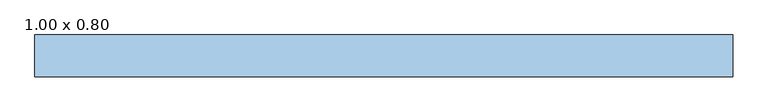
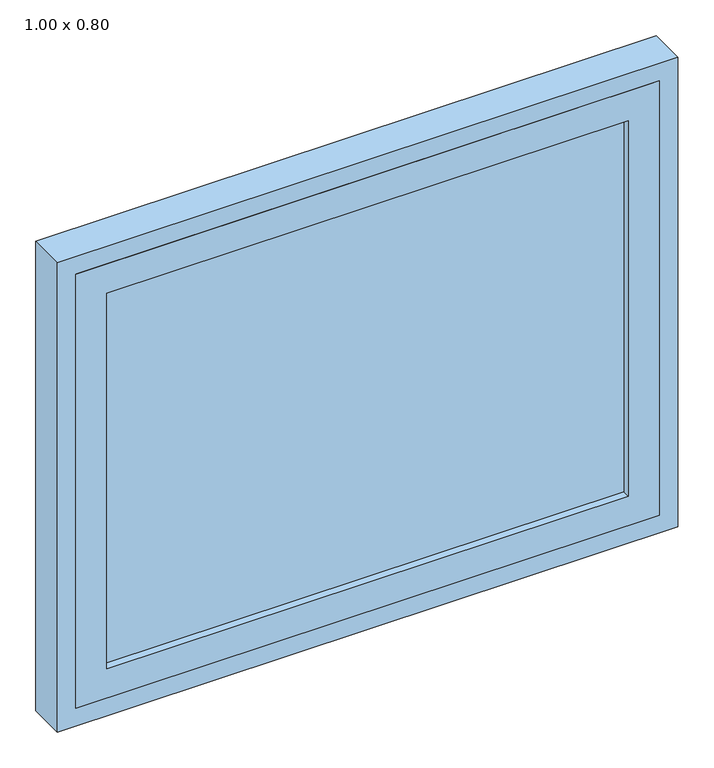
"""IFC4 building model written with IfcOpenShell, lengths in millimetres: window geometry, CC_JANELA MAXIM-AR_1 FOLHA VIDRO : 1.00 x 0.80."""

import ifcopenshell
import ifcopenshell.guid

model = None  # the IFC model being written
_history = None  # IfcOwnerHistory: only IFC2X3 demands one
_inside = {}  # id of a spatial element -> (the spatial element, [elements in it])
_under = {}  # id of a project, library or spatial element -> (it, [spatial elements below it])
_declared = {}  # id of a project -> (the project, [libraries it declares])
_typed = {}  # id of a type object -> (the type object, [elements of that type])
_made_of = {}  # id of a material, layer set ... -> (it, [elements and type objects made of it])


def new_model(schema):
    """Start an empty IFC model of exactly this schema.

    Asked for "IFC4X3", IfcOpenShell would pick the latest addendum, in which some entities
    have other attributes; the version numbers below select the first issue.
    IFC2X3 requires an IfcOwnerHistory on every rooted entity: one is made here for all.
    """
    global model, _history
    if schema == "IFC4X3":
        model = ifcopenshell.file(schema_version=(4, 3, 0, 0))
    else:
        model = ifcopenshell.file(schema=schema)
    _inside.clear()
    _under.clear()
    _declared.clear()
    _typed.clear()
    _made_of.clear()
    _history = None
    if model.schema == "IFC2X3":
        org = make("IfcOrganization", Name="unknown")
        user = make(
            "IfcPersonAndOrganization",
            ThePerson=make("IfcPerson", FamilyName="unknown"),
            TheOrganization=org,
        )
        app = make(
            "IfcApplication",
            ApplicationDeveloper=org,
            Version="unknown",
            ApplicationFullName="unknown",
            ApplicationIdentifier="unknown",
        )
        _history = make(
            "IfcOwnerHistory",
            OwningUser=user,
            OwningApplication=app,
            ChangeAction="ADDED",
            CreationDate=0,
        )
    return model


def make(cls, **values):
    """One entity of the class cls with the attributes given. An attribute that is None is left unset."""
    return model.create_entity(
        cls, **{name: value for name, value in values.items() if value is not None}
    )


def rooted(cls, **values):
    """An entity with a GlobalId (a new one), such as an element, a storey or a relation."""
    return make(cls, GlobalId=ifcopenshell.guid.new(), OwnerHistory=_history, **values)


def si_unit(unit_type, name, prefix=None):
    """IfcSIUnit, for example si_unit("LENGTHUNIT", "METRE", prefix="MILLI")."""
    return make("IfcSIUnit", UnitType=unit_type, Prefix=prefix, Name=name)


def assignment(units):
    """IfcUnitAssignment: the units of a project."""
    return None if units is None else make("IfcUnitAssignment", Units=units)


def point(xyz):
    """IfcCartesianPoint."""
    return None if xyz is None else make("IfcCartesianPoint", Coordinates=xyz)


def direction(xyz):
    """IfcDirection."""
    return None if xyz is None else make("IfcDirection", DirectionRatios=xyz)


def frame(location, z_axis=None, x_axis=None):
    """IfcAxis2Placement3D, a coordinate frame: its origin and axes. An axis left out is left unset."""
    return make(
        "IfcAxis2Placement3D",
        Location=point(location),
        Axis=direction(z_axis),
        RefDirection=direction(x_axis),
    )


def origin():
    """The frame at (0, 0, 0) with its axes left unset."""
    return frame((0.0, 0.0, 0.0))


def place(relative_to, where):
    """IfcLocalPlacement: puts the frame where relative to a parent placement (None: the world)."""
    return make(
        "IfcLocalPlacement", PlacementRelTo=relative_to, RelativePlacement=where
    )


def context(
    kind, dimensions, precision=None, world=None, true_north=None, identifier=None
):
    """IfcGeometricRepresentationContext, for example the 3D "Model" context."""
    return make(
        "IfcGeometricRepresentationContext",
        ContextIdentifier=identifier,
        ContextType=kind,
        CoordinateSpaceDimension=dimensions,
        Precision=precision,
        WorldCoordinateSystem=world,
        TrueNorth=true_north,
    )


def project(units=None, contexts=None):
    """IfcProject with its units and contexts."""
    return rooted(
        "IfcProject",
        Name="project",
        RepresentationContexts=contexts,
        UnitsInContext=assignment(units),
    )


def spatial(cls, under=None, at=None, **own):
    """A site, building, storey or space (cls), placed at a placement, below another one or the project."""
    s = rooted(cls, ObjectPlacement=at, **own)
    if under is not None:
        _under.setdefault(under.id(), (under, []))[1].append(s)
    return s


def polyline(points):
    """IfcPolyline through the points."""
    return make("IfcPolyline", Points=[point(p) for p in points])


def outline(outer, holes=None, kind="AREA"):
    """IfcArbitraryClosedProfileDef: a profile drawn as a closed curve; with holes, ...WithVoids."""
    if holes is None:
        return make("IfcArbitraryClosedProfileDef", ProfileType=kind, OuterCurve=outer)
    return make(
        "IfcArbitraryProfileDefWithVoids",
        ProfileType=kind,
        OuterCurve=outer,
        InnerCurves=holes,
    )


def extrude(swept, where, along, depth):
    """IfcExtrudedAreaSolid: the profile swept, set in the frame where, extruded along a direction by depth."""
    return make(
        "IfcExtrudedAreaSolid",
        SweptArea=swept,
        Position=where,
        ExtrudedDirection=direction(along),
        Depth=depth,
    )


def shape(context_of_items, identifier, shape_type, items):
    """IfcShapeRepresentation: the items that make up one representation, for example the "Body"."""
    return make(
        "IfcShapeRepresentation",
        ContextOfItems=context_of_items,
        RepresentationIdentifier=identifier,
        RepresentationType=shape_type,
        Items=items,
    )


def source(mapping_origin, context_of_items, identifier, shape_type, items):
    """IfcRepresentationMap: a shape defined once, which mapped items show again and again."""
    return make(
        "IfcRepresentationMap",
        MappingOrigin=mapping_origin,
        MappedRepresentation=shape(context_of_items, identifier, shape_type, items),
    )


def transform(
    local_origin,
    x_axis=None,
    y_axis=None,
    z_axis=None,
    scale=None,
    scale2=None,
    scale3=None,
    uniform=True,
):
    """IfcCartesianTransformationOperator3D, or its non-uniform kind. x_axis, y_axis, z_axis: its Axis1, 2, 3."""
    if uniform:
        return make(
            "IfcCartesianTransformationOperator3D",
            Axis1=direction(x_axis),
            Axis2=direction(y_axis),
            LocalOrigin=point(local_origin),
            Scale=scale,
            Axis3=direction(z_axis),
        )
    return make(
        "IfcCartesianTransformationOperator3DnonUniform",
        Axis1=direction(x_axis),
        Axis2=direction(y_axis),
        LocalOrigin=point(local_origin),
        Scale=scale,
        Axis3=direction(z_axis),
        Scale2=scale2,
        Scale3=scale3,
    )


def mapped(mapping_source, mapping_target):
    """IfcMappedItem: shows the shape of a source again, moved by a transform."""
    return make(
        "IfcMappedItem", MappingSource=mapping_source, MappingTarget=mapping_target
    )


def made_of(thing, what):
    """Note that an element or type object is made of a material, layer set ...; save() writes the relation."""
    if what is not None:
        _made_of.setdefault(what.id(), (what, []))[1].append(thing)
    return thing


def element(
    cls,
    number,
    at=None,
    inside=None,
    cuts=None,
    type_object=None,
    material=None,
    context=None,
    identifier="Body",
    shape_type=None,
    held_by="IfcProductDefinitionShape",
    body=None,
    shapes=None,
    **own,
):
    """One element of the class cls, such as IfcWall. Its Tag is "e" and its number.

    at: its placement. inside: the storey or other place that contains it. cuts: it is an
    opening in that element (IfcRelVoidsElement). A single representation is given by context,
    identifier, shape_type and body (its items); several are given by shapes. held_by: the class
    of the entity that holds the representations. save() writes the other relations.
    """
    e = rooted(cls, Tag="e%d" % number, ObjectPlacement=at, **own)
    if body is not None:
        shapes = [shape(context, identifier, shape_type, body)]
    if shapes is not None:
        e.Representation = make(held_by, Representations=shapes)
    if inside is not None:
        _inside.setdefault(inside.id(), (inside, []))[1].append(e)
    if cuts is not None:
        rooted(
            "IfcRelVoidsElement", RelatingBuildingElement=cuts, RelatedOpeningElement=e
        )
    if type_object is not None:
        _typed.setdefault(type_object.id(), (type_object, []))[1].append(e)
    return made_of(e, material)


def aggregate(whole, parts):
    """IfcRelAggregates: a whole, such as a stair, and the parts it consists of."""
    return rooted("IfcRelAggregates", RelatingObject=whole, RelatedObjects=parts)


def save(model, path):
    """Write the relations noted so far, then the file.

    IfcRelAggregates (storeys below a building ...), IfcRelContainedInSpatialStructure (elements
    in a storey), IfcRelDefinesByType, IfcRelAssociatesMaterial and IfcRelDeclares: one each for
    every whole, place, type object, material and project.
    """
    for whole, parts in _under.values():
        aggregate(whole, parts)
    for where, things in _inside.values():
        rooted(
            "IfcRelContainedInSpatialStructure",
            RelatedElements=things,
            RelatingStructure=where,
        )
    for kind, things in _typed.values():
        rooted("IfcRelDefinesByType", RelatedObjects=things, RelatingType=kind)
    for what, things in _made_of.values():
        rooted("IfcRelAssociatesMaterial", RelatedObjects=things, RelatingMaterial=what)
    for by, libraries in _declared.values():
        rooted("IfcRelDeclares", RelatingContext=by, RelatedDefinitions=libraries)
    model.write(path)


def window_1_00_x_0_80_3e14d2bc(model_context):
    return source(origin(), model_context, "Body", "SweptSolid", [
        extrude(outline(polyline([(-420.0, -87.5), (-420.0, -82.5), (420.0, -82.5), (420.0, -87.5), (-420.0, -87.5)])), frame((0.0, 0.0, 1780.0), z_axis=(0.0, 0.0, 1.0), x_axis=(1.0, 0.0, 0.0)), (0.0, 0.0, 1.0), 640.0),
        extrude(outline(polyline([(2470.0, -470.0), (1730.0, -470.0), (1730.0, 470.0), (2470.0, 470.0), (2470.0, -470.0)]), holes=[polyline([(2420.0, 420.0), (1780.0, 420.0), (1780.0, -420.0), (2420.0, -420.0), (2420.0, 420.0)])]), frame((0.0, -100.0, 0.0), z_axis=(0.0, 1.0, 0.0), x_axis=(0.0, 0.0, 1.0)), (0.0, 0.0, 1.0), 30.0),
        extrude(outline(polyline([(1700.0, 500.0), (2500.0, 500.0), (2500.0, -500.0), (1700.0, -500.0), (1700.0, 500.0)]), holes=[polyline([(1730.0, -470.0), (2470.0, -470.0), (2470.0, 470.0), (1730.0, 470.0), (1730.0, -470.0)])]), frame((0.0, -100.0, 0.0), z_axis=(0.0, 1.0, 0.0), x_axis=(0.0, 0.0, 1.0)), (0.0, 0.0, 1.0), 60.0),
    ])


if __name__ == "__main__":
    model = new_model("IFC4")
    model_context = context("Model", 3, world=origin())
    ifc_project = project(units=[si_unit("LENGTHUNIT", "METRE", prefix="MILLI")], contexts=[model_context])
    site = spatial("IfcSite", under=ifc_project)
    building = spatial("IfcBuilding", under=site)
    placement = place(None, origin())
    window_1_00_x_0_80_shape = window_1_00_x_0_80_3e14d2bc(model_context)
    element("IfcWindow", 1, ObjectType="CC_JANELA MAXIM-AR_1 FOLHA VIDRO : 1.00 x 0.80", at=placement, inside=building, context=model_context, shape_type="MappedRepresentation", body=[
        mapped(window_1_00_x_0_80_shape, transform((0.0, 0.0, 0.0), x_axis=(1.0, 0.0, 0.0), y_axis=(0.0, 1.0, 0.0), z_axis=(0.0, 0.0, 1.0))),
    ])
    save(model, "model.ifc")

# Revit data of these elements
# Type "CC_JANELA MAXIM-AR_1 FOLHA VIDRO : 1.00 x 0.80"
#   Type Mark = "J7"
#   Site = "www.construir.arq.br"
#   Empresa = "Cursos Construir"
#   Description = "JANELA MAXIM-AR 1 FOLHA VIDRO"
#   Criado Por = "Roberto Netto"
#   Analytic Construction = "<Nenhum>"
#   Atualizado por = "Rudemberg Eloi"
#   Rough Width = 1.00 m
#   Largura Moldura Folha [instance default] = 0.05 m
#   Largura Moldura Externa [instance default] = 0.10 m
#   Largura Guarnição Interna [instance default] = 0.05 m
#   Largura Folha [instance default] = 0.94 m
#   Interna [instance default] = 0.00 m
#   Externa [instance default] = 0.00 m
#   Extensão Frontal Peitoril/Pngadeira [instance default] = 0.03 m
#   Extensão Exterior Direita Peitoril/Pingadeira [instance default] = 0.025 m
#   Extensão Caixilho [instance default] = 0.03 m
#   Extensâo Exterior Esquerda Peitoril/Pingadeira [instance default] = 0.025 m
#   Espessura Peitoril/Pingadeira [instance default] = 0.02 m
#   Espessura Moldura Externa [instance default] = 0.01 m
#   Espessura Guarnição Interna [instance default] = 0.005 m
#   Espessura Folha [instance default] = 0.03 m
#   Espessura Caixilho [instance default] = 0.03 m
#   Cálculo Abertura Linear [instance default] = 0.00 m
#   Rough Height = 0.80 m
#   Altura Folha [instance default] = 0.74 m
#   Altura Corte [instance default] = 0.02 m
#   Height = 0.80 m
#   Width = 1.00 m
#   ----PEITORIL/PINGADEIRA---- [instance default] = 0.00 m
#   ----MOLDURA---- [instance default] = 0.00 m
#   ----GUARNIÇÃO---- [instance default] = 0.00 m
#   ----FOLHA---- [instance default] = 0.00 m
#   ----EXTENSÃO---- [instance default] = 0.00 m
#   ----CAIXILHO---- [instance default] = 0.00 m
#   Peitoril/Pingadeira Vazio [instance default] = no
#   Peitoril/Pingadeira Família [instance default] = yes
#   Moldura Externa [instance default] = no
#   Guarnição Interna [instance default] = yes
#   Material Vidro Folha = .VIDRO
#   Material Peitoril/Pingadeira = .GRANITO BRANCO ITAÚNAS
#   Material Moldura Folha = .ALUMÍNIO COM PINTURA ELETROSTÁTICA BRANCA
#   Material Moldura Externa = .PINTURA ACRÍLICA BRANCA
#   Material Guarnição = .ALUMÍNIO COM PINTURA ELETROSTÁTICA BRANCA
#   Material Caixilho = .ALUMÍNIO COM PINTURA ELETROSTÁTICA BRANCA
#   Wall Closure = (empty or 0)
# Element 1 (IfcWindow, "CC_JANELA MAXIM-AR_1 FOLHA VIDRO : 1.00 x 0.80")
#   Guarnição Interna = no
#   Materials on its faces: ".ALUMÍNIO COM PINTURA ELETROSTÁTICA BRANCA", ".VIDRO"
# Materials
#   ".VIDRO": class "Genérico", colour RGB 198 236 255, transparency 0.95, Cost = 0
#   ".GRANITO BRANCO ITAÚNAS": class ".CC_PEDRA REVEST.", colour RGB 202 195 174, transparency 0, Description = "Granito branco Itaúnas", Uso = "Pedra", Cost = 0
#   ".ALUMÍNIO COM PINTURA ELETROSTÁTICA BRANCA": class "CC_METAIS", colour RGB 241 241 241, transparency 0, Cost = 0
#   ".PINTURA ACRÍLICA BRANCA": class ".CC_PINTURA", colour RGB 250 250 250, transparency 0, Keynote = "09910.A1", Description = "Tinta acrílica na cor branca", Cost = 0
